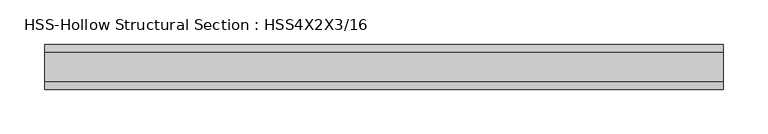
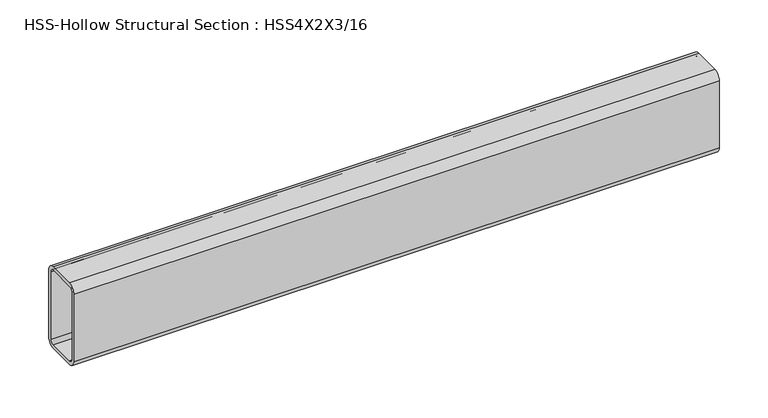
"""IFC4 building model written with IfcOpenShell, lengths in millimetres: beam geometry, HSS-Hollow Structural Section : HSS4X2X3/16."""

from ifc_helpers import new_model, si_unit, point, frame, frame_2d, origin, place, context, project, spatial, polyline, circle_curve, trimmed, segment, composite_curve, outline, extrude, source, transform, mapped, element, save


def hss_hollow_structural_section_hss4x2x3_16_afd03f9b(model_context):
    return source(origin(), model_context, "Body", "SweptSolid", [
        extrude(outline(composite_curve([segment(polyline([(25.4, 41.9608), (25.4, -41.9608)]), True, "CONTINUOUS"), segment(trimmed(circle_curve(frame_2d((16.5608, -41.9608)), 8.8392), [point((25.4, -41.9608))], [point((16.5608, -50.8))], False, "CARTESIAN"), True, "CONTINUOUS"), segment(polyline([(16.5608, -50.8), (-16.5608, -50.8)]), True, "CONTINUOUS"), segment(trimmed(circle_curve(frame_2d((-16.5608, -41.9608)), 8.8392), [point((-16.5608, -50.8))], [point((-25.4, -41.9608))], False, "CARTESIAN"), True, "CONTINUOUS"), segment(polyline([(-25.4, -41.9608), (-25.4, 41.9608)]), True, "CONTINUOUS"), segment(trimmed(circle_curve(frame_2d((-16.5608, 41.9608)), 8.8392), [point((-25.4, 41.9608))], [point((-16.5608, 50.8))], False, "CARTESIAN"), True, "CONTINUOUS"), segment(polyline([(-16.5608, 50.8), (16.5608, 50.8)]), True, "CONTINUOUS"), segment(trimmed(circle_curve(frame_2d((16.5608, 41.9608)), 8.8392), [point((16.5608, 50.8))], [point((25.4, 41.9608))], False, "CARTESIAN"), True, "CONTINUOUS")], self_intersect=False), holes=[composite_curve([segment(trimmed(circle_curve(frame_2d((-16.5608, 41.9608)), 4.4196), [point((-16.5608, 46.3804))], [point((-20.9804, 41.9608))], True, "CARTESIAN"), True, "CONTINUOUS"), segment(polyline([(-20.9804, 41.9608), (-20.9804, -41.9608)]), True, "CONTINUOUS"), segment(trimmed(circle_curve(frame_2d((-16.5608, -41.9608)), 4.4196), [point((-20.9804, -41.9608))], [point((-16.5608, -46.3804))], True, "CARTESIAN"), True, "CONTINUOUS"), segment(polyline([(-16.5608, -46.3804), (16.5608, -46.3804)]), True, "CONTINUOUS"), segment(trimmed(circle_curve(frame_2d((16.5608, -41.9608)), 4.4196), [point((16.5608, -46.3804))], [point((20.9804, -41.9608))], True, "CARTESIAN"), True, "CONTINUOUS"), segment(polyline([(20.9804, -41.9608), (20.9804, 41.9608)]), True, "CONTINUOUS"), segment(trimmed(circle_curve(frame_2d((16.5608, 41.9608)), 4.4196), [point((20.9804, 41.9608))], [point((16.5608, 46.3804))], True, "CARTESIAN"), True, "CONTINUOUS"), segment(polyline([(16.5608, 46.3804), (-16.5608, 46.3804)]), True, "CONTINUOUS")], self_intersect=False)]), frame((-381.0, 0.0, 0.0), z_axis=(1.0, 0.0, 0.0), x_axis=(0.0, 1.0, 0.0)), (0.0, 0.0, 1.0), 762.0),
    ])


if __name__ == "__main__":
    model = new_model("IFC4")
    model_context = context("Model", 3, world=origin())
    ifc_project = project(units=[si_unit("LENGTHUNIT", "METRE", prefix="MILLI")], contexts=[model_context])
    site = spatial("IfcSite", under=ifc_project)
    building = spatial("IfcBuilding", under=site)
    placement = place(None, origin())
    hss_hollow_structural_section_hss4x2x3_16_shape = hss_hollow_structural_section_hss4x2x3_16_afd03f9b(model_context)
    element("IfcBeam", 1, ObjectType="HSS-Hollow Structural Section : HSS4X2X3/16", at=placement, inside=building, context=model_context, shape_type="MappedRepresentation", body=[
        mapped(hss_hollow_structural_section_hss4x2x3_16_shape, transform((0.0, 0.0, 0.0), x_axis=(1.0, 0.0, 0.0), y_axis=(0.0, 1.0, 0.0), z_axis=(0.0, 0.0, 1.0))),
    ])
    save(model, "model.ifc")

# Revit data of these elements
# Type "HSS-Hollow Structural Section : HSS4X2X3/16"
#   Assembly Code = "B10"
#   Shape = "Rect."
#   W = 6.87
#   Ht = 0' - 4"
#   Length [instance default] = 5' - 0"
#   b = 0' - 2"
#   kr = 0' - 0.348"
#   t = 0' - 0.174"
#   A = 0.013125 SF
#   Structural Material [instance default] = none
